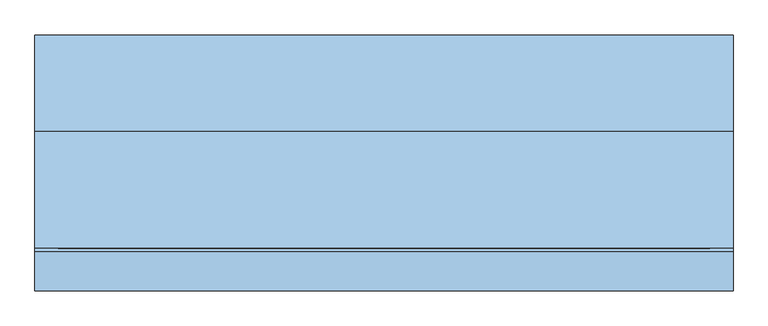
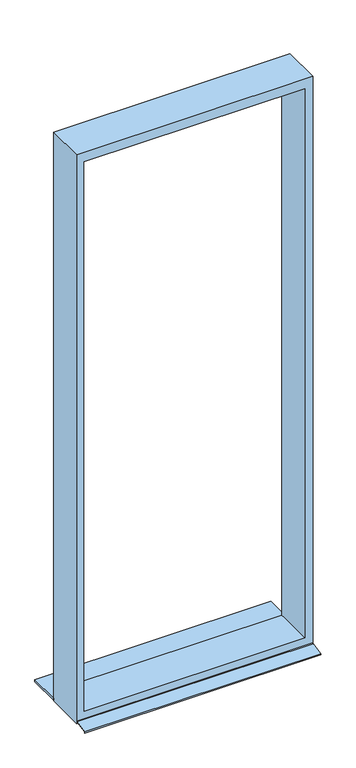
"""IFC4 building model written with IfcOpenShell, lengths in millimetres: window geometry, Fenster - Festverglasung : Feste Verglasung 4.58 x 1.8."""

from ifc_helpers import new_model, si_unit, frame, origin, place, context, project, spatial, polyline, outline, extrude, source, transform, mapped, element, save


def window_096931ef(model_context):
    return source(origin(), model_context, "Body", "SweptSolid", [
        extrude(outline(polyline([(5580.0, 900.0), (5580.0, -900.0), (1000.0, -900.0), (1000.0, 900.0), (5580.0, 900.0)]), holes=[polyline([(5500.0, 840.0), (1080.0, 840.0), (1080.0, -840.0), (5500.0, -840.0), (5500.0, 840.0)])]), frame((0.0, -220.0, 0.0), z_axis=(0.0, 1.0, 0.0), x_axis=(0.0, 0.0, 1.0)), (0.0, 0.0, 1.0), 300.0),
        extrude(outline(polyline([(-900.0, 330.0), (900.0, 330.0), (900.0, 80.0), (-900.0, 80.0), (-900.0, 330.0)])), frame((0.0, 0.0, 1005.0), z_axis=(0.0, 0.0, 1.0), x_axis=(1.0, 0.0, 0.0)), (0.0, 0.0, 1.0), 15.0),
        extrude(outline(polyline([(-230.0221543, 1020.0), (-220.0, 1020.0), (-220.0, 1018.0), (-229.8240723, 1018.0), (-328.0, 998.3604634), (-328.0, 990.0), (-330.0, 990.0), (-330.0, 1000.0), (-230.0221543, 1020.0)])), frame((-900.0, 0.0, 0.0), z_axis=(1.0, 0.0, 0.0), x_axis=(0.0, 1.0, 0.0)), (0.0, 0.0, 1.0), 1800.0),
    ])


if __name__ == "__main__":
    model = new_model("IFC4")
    model_context = context("Model", 3, world=origin())
    ifc_project = project(units=[si_unit("LENGTHUNIT", "METRE", prefix="MILLI")], contexts=[model_context])
    site = spatial("IfcSite", under=ifc_project)
    building = spatial("IfcBuilding", under=site)
    placement = place(None, origin())
    window_shape = window_096931ef(model_context)
    element("IfcWindow", 1, ObjectType="Fenster - Festverglasung : Feste Verglasung 4.58 x 1.8", at=placement, inside=building, context=model_context, shape_type="MappedRepresentation", body=[
        mapped(window_shape, transform((0.0, 0.0, 0.0), x_axis=(1.0, 0.0, 0.0), y_axis=(0.0, 1.0, 0.0), z_axis=(0.0, 0.0, 1.0))),
    ])
    save(model, "model.ifc")

# Revit data of these elements
# Type "Fenster - Festverglasung : Feste Verglasung 4.58 x 1.8"
#   Type Mark = "52"
#   Operation = "SinglePanel"
#   Keynote = "16.05.01"
#   Visual Light Transmittance = 0.9
#   Solar Heat Gain Coefficient = 0.78
#   Rough Width = 1.800 m
#   Rough Height = 4.580 m
#   Heat Transfer Coefficient (U) = 3.6886 W/(m²·K)
#   Rahmentiefe = 0.300 m
#   Rahmenhöhe unten = 0.080 m
#   Höhe oberer  Rahmen = 0.080 m
#   Rahmenbreite = 0.060 m
#   Height = 4.580 m
#   Einbautiefe (von außen) [instance default] = 0.080 m
#   Width = 1.800 m
#   Wall Closure = 3
#   Bild [instance default] = none
#   Glas [instance default] = none
#   Innere Fensterbank [instance default] = none
#   Äußere Fensterbank [instance default] = none
#   Construction Type Id = ""
#   Analytic Construction = (empty or 0)
# Element 1 (IfcWindow, "Fenster - Festverglasung : Feste Verglasung 4.58 x 1.8")
#   Materials on its faces: "Kunststoff - Weiß", "Holz - Birke"
# Materials
#   "Kunststoff - Weiß": class "Kunststoff", colour RGB 249 249 249, transparency 0, Cost = 0
#   "Holz - Birke": class "Holz", colour RGB 213 164 103, transparency 0, Cost = 0
